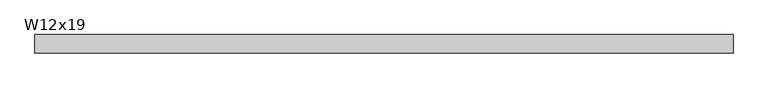
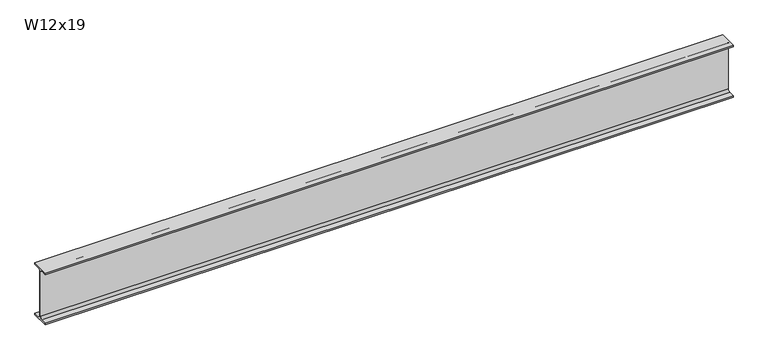
"""IFC4 building model written with IfcOpenShell, lengths in millimetres: beam geometry, RME W-Wide Flange : W12x19."""

from ifc_helpers import new_model, si_unit, point, frame, frame_2d, origin, place, context, project, spatial, polyline, circle_curve, trimmed, segment, composite_curve, outline, extrude, source, transform, mapped, element, save


def w12x19_982e5906(model_context):
    return source(origin(), model_context, "Body", "SweptSolid", [
        extrude(outline(composite_curve([segment(polyline([(50.927, -146.05), (50.927, -154.94), (-50.927, -154.94), (-50.927, -146.05), (-16.3195, -146.05)]), True, "CONTINUOUS"), segment(trimmed(circle_curve(frame_2d((-16.3195, -132.715)), 13.335), [point((-16.3195, -146.05))], [point((-2.9845, -132.715))], True, "CARTESIAN"), True, "CONTINUOUS"), segment(polyline([(-2.9845, -132.715), (-2.9845, 132.715)]), True, "CONTINUOUS"), segment(trimmed(circle_curve(frame_2d((-16.3195, 132.715)), 13.335), [point((-2.9845, 132.715))], [point((-16.3195, 146.05))], True, "CARTESIAN"), True, "CONTINUOUS"), segment(polyline([(-16.3195, 146.05), (-50.927, 146.05), (-50.927, 154.94), (50.927, 154.94), (50.927, 146.05), (16.3195, 146.05)]), True, "CONTINUOUS"), segment(trimmed(circle_curve(frame_2d((16.3195, 132.715)), 13.335), [point((16.3195, 146.05))], [point((2.9845, 132.715))], True, "CARTESIAN"), True, "CONTINUOUS"), segment(polyline([(2.9845, 132.715), (2.9845, -132.715)]), True, "CONTINUOUS"), segment(trimmed(circle_curve(frame_2d((16.3195, -132.715)), 13.335), [point((2.9845, -132.715))], [point((16.3195, -146.05))], True, "CARTESIAN"), True, "CONTINUOUS"), segment(polyline([(16.3195, -146.05), (50.927, -146.05)]), True, "CONTINUOUS")], self_intersect=False)), frame((-1931.67, 0.0, 0.0), z_axis=(1.0, 0.0, 0.0), x_axis=(0.0, 1.0, 0.0)), (0.0, 0.0, 1.0), 3883.152),
    ])


if __name__ == "__main__":
    model = new_model("IFC4")
    model_context = context("Model", 3, world=origin())
    ifc_project = project(units=[si_unit("LENGTHUNIT", "METRE", prefix="MILLI")], contexts=[model_context])
    site = spatial("IfcSite", under=ifc_project)
    building = spatial("IfcBuilding", under=site)
    placement = place(None, origin())
    w12x19_shape = w12x19_982e5906(model_context)
    element("IfcBeam", 1, ObjectType="RME W-Wide Flange : W12x19", at=placement, inside=building, context=model_context, shape_type="MappedRepresentation", body=[
        mapped(w12x19_shape, transform((0.0, 0.0, 0.0), x_axis=(1.0, 0.0, 0.0), y_axis=(0.0, 1.0, 0.0), z_axis=(0.0, 0.0, 1.0))),
    ])
    save(model, "model.ifc")

# Revit data of these elements
# Type "RME W-Wide Flange : W12x19"
#   WELD P [instance default] = ""
#   WELD LE [instance default] = ""
#   WELD D [instance default] = ""
#   TOP SECTION SIZE [instance default] = ""
#   TOP SECTION LENGTH [instance default] = ""
#   REMARKS [instance default] = ""
#   REINF TYPE [instance default] = ""
#   Nominal Size = "W24"
#   End Bearing Capacity [instance default] = ""
#   BOT SECTION SIZE [instance default] = ""
#   BOT SECTION LENGTH [instance default] = ""
#   Assembly Code = "B10"
#   W = 19
#   Start Extension Calculation [instance default] = 10' - 0"
#   Start Extension [instance default] = -0' - 0 1/2"
#   End Extension Calculation [instance default] = 10' - 0"
#   End Extension [instance default] = -0' - 0 1/2"
#   Length [instance default] = 5' - 0"
#   bf = 0' - 4.01"
#   d = 1' - 0.2"
#   k = 0' - 0 7/8"
#   k2 = 0' - 0.525"
#   tf = 0' - 0.35"
#   tw = 0' - 0.235"
#   A = 0.0386806 SF
#   Structural Material [instance default] = Metal - Steel - ASTM A992
# Element 1 (IfcBeam, "RME W-Wide Flange : W12x19")
#   Length = 13' - 5.16"
#   Materials on its faces: "Metal - Steel - ASTM A992"
# Materials
#   "Metal - Steel - ASTM A992": class "Metal", colour RGB 255 128 0, transparency 0
